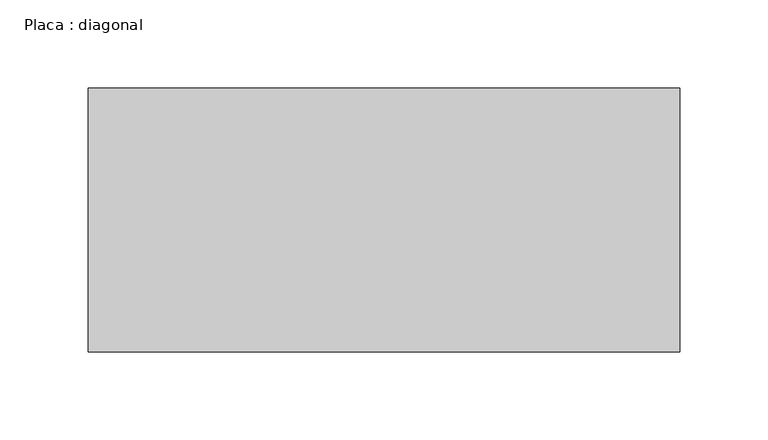
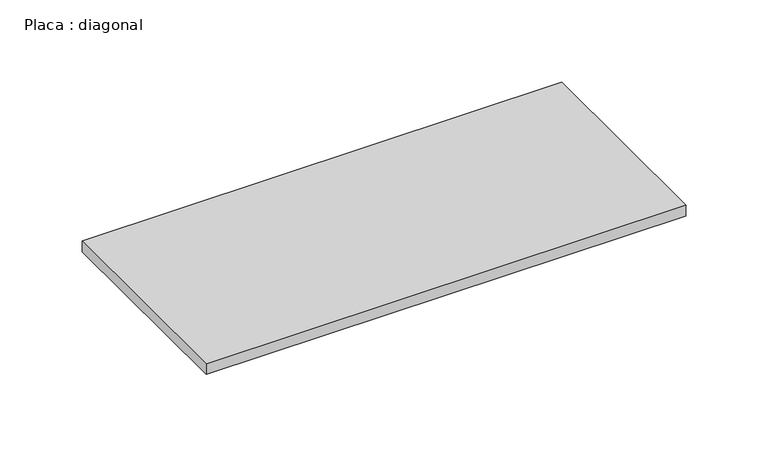
"""IFC4 building model written with IfcOpenShell, lengths in millimetres: beam geometry, Placa : diagonal."""

from ifc_helpers import new_model, si_unit, frame, origin, place, context, project, spatial, polyline, outline, extrude, source, transform, mapped, element, save


def placa_diagonal_3ead9384(model_context):
    return source(origin(), model_context, "Body", "SweptSolid", [
        extrude(outline(polyline([(168.0075509, 75.0), (168.0075509, -75.0), (-168.0075509, -75.0), (-168.0075509, 75.0), (168.0075509, 75.0)])), frame((0.0, 0.0, -4.0), z_axis=(0.0, 0.0, 1.0), x_axis=(1.0, 0.0, 0.0)), (0.0, 0.0, 1.0), 8.0),
    ])


if __name__ == "__main__":
    model = new_model("IFC4")
    model_context = context("Model", 3, world=origin())
    ifc_project = project(units=[si_unit("LENGTHUNIT", "METRE", prefix="MILLI")], contexts=[model_context])
    site = spatial("IfcSite", under=ifc_project)
    building = spatial("IfcBuilding", under=site)
    placement = place(None, origin())
    placa_diagonal_shape = placa_diagonal_3ead9384(model_context)
    element("IfcBeam", 1, ObjectType="Placa : diagonal", at=placement, inside=building, context=model_context, shape_type="MappedRepresentation", body=[
        mapped(placa_diagonal_shape, transform((0.0, 0.0, 0.0), x_axis=(1.0, 0.0, 0.0), y_axis=(0.0, 1.0, 0.0), z_axis=(0.0, 0.0, 1.0))),
    ])
    save(model, "model.ifc")

# Revit data of these elements
# Type "Placa : diagonal"
#   W = 0
#   Length [instance default] = 1.50 m
#   b = 0.15 m
#   d = 0.008 m
#   A = 0 m²
#   Structural Material [instance default] = Aço, 45-345
# Element 1 (IfcBeam, "Placa : diagonal")
#   Materials on its faces: "Aço, 45-345"
# Materials
#   "Aço, 45-345": class "Metal", colour RGB 247 247 247, transparency 0, Description = "Aço 345 MPa", Cost = 0
